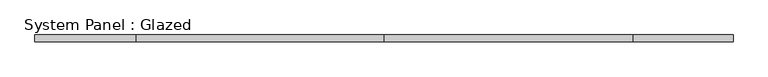
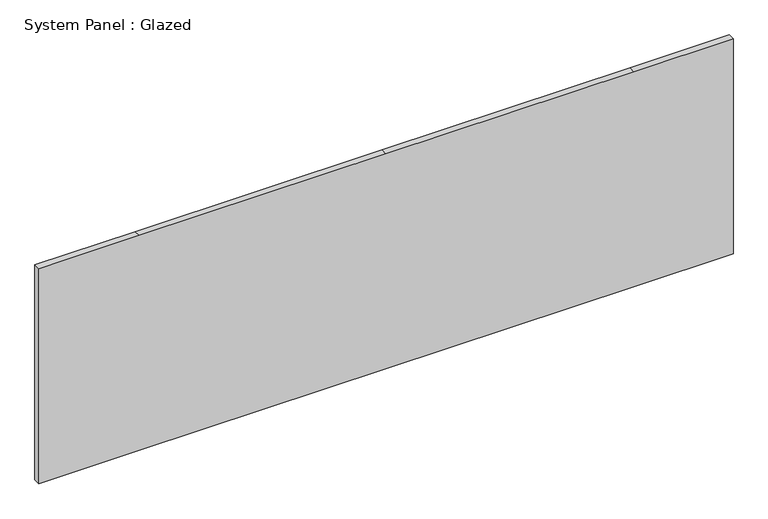
"""IFC4 building model written with IfcOpenShell, lengths in millimetres: plate geometry, System Panel : Glazed."""

from ifc_helpers import new_model, si_unit, frame, origin, place, context, project, spatial, polyline, outline, extrude, source, transform, mapped, element, save


def system_panel_glazed_db96f60a(model_context):
    return source(origin(), model_context, "Body", "SweptSolid", [
        extrude(outline(polyline([(0.0, -1328.0571429), (0.0, -943.4285714), (0.0, 0.0), (0.0, 948.8714286), (0.0, 1328.0571429), (869.95, 1328.0571429), (869.95, 948.8714286), (869.95, 0.0), (869.95, -943.4285714), (869.95, -1328.0571429), (0.0, -1328.0571429)])), frame((0.0, 19.05, 0.0), z_axis=(0.0, 1.0, 0.0), x_axis=(0.0, 0.0, 1.0)), (0.0, 0.0, 1.0), 25.4),
    ])


if __name__ == "__main__":
    model = new_model("IFC4")
    model_context = context("Model", 3, world=origin())
    ifc_project = project(units=[si_unit("LENGTHUNIT", "METRE", prefix="MILLI")], contexts=[model_context])
    site = spatial("IfcSite", under=ifc_project)
    building = spatial("IfcBuilding", under=site)
    placement = place(None, origin())
    system_panel_glazed_shape = system_panel_glazed_db96f60a(model_context)
    element("IfcPlate", 1, ObjectType="System Panel : Glazed", at=placement, inside=building, context=model_context, shape_type="MappedRepresentation", body=[
        mapped(system_panel_glazed_shape, transform((0.0, 0.0, 0.0), x_axis=(1.0, 0.0, 0.0), y_axis=(0.0, 1.0, 0.0), z_axis=(0.0, 0.0, 1.0))),
    ])
    save(model, "model.ifc")

# Revit data of these elements
# Element 1 (IfcPlate, "System Panel : Glazed")
#   Materials on its faces: "Glass"
# Materials
#   "Glass": class "Glass", colour RGB 0 128 192, transparency 0.75
